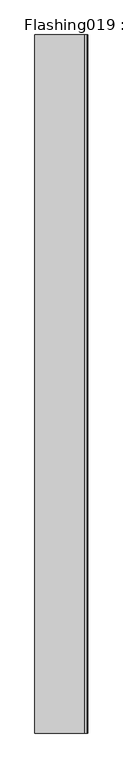
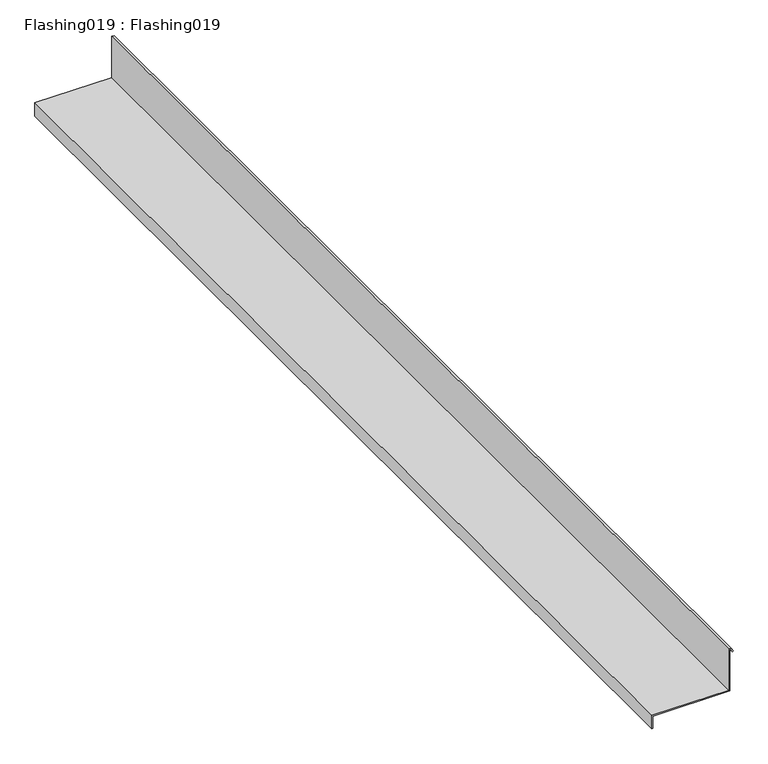
"""IFC4 building model written with IfcOpenShell, lengths in millimetres: proxy geometry, Flashing019 : Flashing019."""

from ifc_helpers import new_model, si_unit, frame, origin, place, context, project, spatial, polyline, outline, extrude, source, transform, mapped, element, save


def flashing019_flashing019_9dc0ec64(model_context):
    return source(origin(), model_context, "Body", "SweptSolid", [
        extrude(outline(polyline([(40784.7382813, 16649.96875), (40784.7382813, 16645.2851562), (40703.2466161, 16645.2851562), (40703.2466161, 16501.84375), (40677.1179688, 16501.84375), (40677.1179688, 16503.84375), (40701.2466161, 16503.84375), (40701.2466161, 16647.2851563), (40782.7382813, 16647.2851563), (40782.7382813, 16648.7903893), (40776.8666698, 16652.0435345), (40777.8359375, 16653.7929687), (40784.7382813, 16649.96875)])), frame((0.0, 7982.1449366, 0.0), z_axis=(0.0, 1.0, 0.0), x_axis=(0.0, 0.0, 1.0)), (0.0, 0.0, 1.0), 2000.0),
    ])


if __name__ == "__main__":
    model = new_model("IFC4")
    model_context = context("Model", 3, world=origin())
    ifc_project = project(units=[si_unit("LENGTHUNIT", "METRE", prefix="MILLI")], contexts=[model_context])
    site = spatial("IfcSite", under=ifc_project)
    building = spatial("IfcBuilding", under=site)
    placement = place(None, origin())
    flashing019_flashing019_shape = flashing019_flashing019_9dc0ec64(model_context)
    element("IfcBuildingElementProxy", 1, Name="Flashing019 : Flashing019", ObjectType="Flashing019 : Flashing019", at=placement, inside=building, context=model_context, shape_type="MappedRepresentation", body=[
        mapped(flashing019_flashing019_shape, transform((0.0, 0.0, 0.0), x_axis=(1.0, 0.0, 0.0), y_axis=(0.0, 1.0, 0.0), z_axis=(0.0, 0.0, 1.0))),
    ])
    save(model, "model.ifc")

# Revit data of these elements
# Type "Flashing019 : Flashing019"
#   NameOverride = "Flashing019"
# Element 1 (IfcBuildingElementProxy, "Flashing019 : Flashing019")
#   Materials on its faces: "BRAKE METAL TO WRAP FRAMING OVER BITUTHANE"
# Materials
#   "BRAKE METAL TO WRAP FRAMING OVER BITUTHANE": class "Unassigned", colour RGB 128 128 128, transparency 0, Cost = 0
